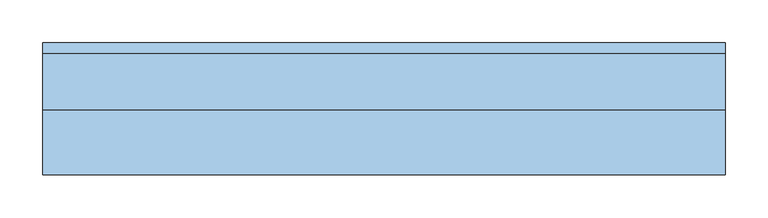
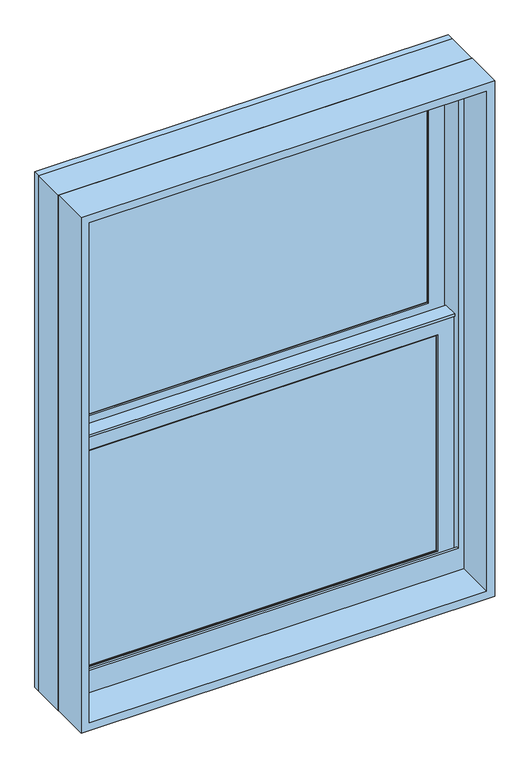
"""IFC4 building model written with IfcOpenShell, lengths in millimetres: window geometry, Window-Double_Hung-Marvin-Essential : ESDH2836."""

from ifc_helpers import new_model, si_unit, frame, origin, place, context, project, spatial, polyline, outline, extrude, faceted_brep, source, transform, mapped, element, save


def window_51e557a5(model_context):
    return source(origin(), model_context, "Body", "SolidModel", [
        extrude(outline(polyline([(123.825, 20.6375), (123.825, 15.875), (104.775, 15.875), (104.775, 20.6375), (123.825, 20.6375)])), frame((0.0, 0.0, 1441.45), z_axis=(0.0, 0.0, 1.0), x_axis=(1.0, 0.0, 0.0)), (0.0, 0.0, 1.0), 450.85),
        extrude(outline(polyline([(-104.775, 20.6375), (-104.775, 15.875), (-123.825, 15.875), (-123.825, 20.6375), (-104.775, 20.6375)])), frame((0.0, 0.0, 1441.45), z_axis=(0.0, 0.0, 1.0), x_axis=(1.0, 0.0, 0.0)), (0.0, 0.0, 1.0), 450.85),
        extrude(outline(polyline([(342.9, 20.6375), (342.9, 15.875), (-342.9, 15.875), (-342.9, 20.6375), (342.9, 20.6375)])), frame((0.0, 0.0, 1657.35), z_axis=(0.0, 0.0, 1.0), x_axis=(1.0, 0.0, 0.0)), (0.0, 0.0, 1.0), 19.05),
        extrude(outline(polyline([(-123.825, 46.83125), (-123.825, 51.59375), (-104.775, 51.59375), (-104.775, 46.83125), (-123.825, 46.83125)])), frame((0.0, 0.0, 1930.4), z_axis=(0.0, 0.0, 1.0), x_axis=(1.0, 0.0, 0.0)), (0.0, 0.0, 1.0), 450.85),
        extrude(outline(polyline([(104.775, 46.83125), (104.775, 51.59375), (123.825, 51.59375), (123.825, 46.83125), (104.775, 46.83125)])), frame((0.0, 0.0, 1930.4), z_axis=(0.0, 0.0, 1.0), x_axis=(1.0, 0.0, 0.0)), (0.0, 0.0, 1.0), 450.85),
        extrude(outline(polyline([(-342.9, 46.83125), (-342.9, 51.59375), (342.9, 51.59375), (342.9, 46.83125), (-342.9, 46.83125)])), frame((0.0, 0.0, 2146.3), z_axis=(0.0, 0.0, 1.0), x_axis=(1.0, 0.0, 0.0)), (0.0, 0.0, 1.0), 19.05),
        extrude(outline(polyline([(123.825, 20.6375), (104.775, 20.6375), (104.775, 25.4), (123.825, 25.4), (123.825, 20.6375)])), frame((0.0, 0.0, 1441.45), z_axis=(0.0, 0.0, 1.0), x_axis=(1.0, 0.0, 0.0)), (0.0, 0.0, 1.0), 450.85),
        extrude(outline(polyline([(-104.775, 20.6375), (-123.825, 20.6375), (-123.825, 25.4), (-104.775, 25.4), (-104.775, 20.6375)])), frame((0.0, 0.0, 1441.45), z_axis=(0.0, 0.0, 1.0), x_axis=(1.0, 0.0, 0.0)), (0.0, 0.0, 1.0), 450.85),
        extrude(outline(polyline([(342.9, 20.6375), (-342.9, 20.6375), (-342.9, 25.4), (342.9, 25.4), (342.9, 20.6375)])), frame((0.0, 0.0, 1657.35), z_axis=(0.0, 0.0, 1.0), x_axis=(1.0, 0.0, 0.0)), (0.0, 0.0, 1.0), 19.05),
        extrude(outline(polyline([(-123.825, 56.35625), (-104.775, 56.35625), (-104.775, 51.59375), (-123.825, 51.59375), (-123.825, 56.35625)])), frame((0.0, 0.0, 1930.4), z_axis=(0.0, 0.0, 1.0), x_axis=(1.0, 0.0, 0.0)), (0.0, 0.0, 1.0), 450.85),
        extrude(outline(polyline([(104.775, 56.35625), (123.825, 56.35625), (123.825, 51.59375), (104.775, 51.59375), (104.775, 56.35625)])), frame((0.0, 0.0, 1930.4), z_axis=(0.0, 0.0, 1.0), x_axis=(1.0, 0.0, 0.0)), (0.0, 0.0, 1.0), 450.85),
        extrude(outline(polyline([(-342.9, 56.35625), (342.9, 56.35625), (342.9, 51.59375), (-342.9, 51.59375), (-342.9, 56.35625)])), frame((0.0, 0.0, 2146.3), z_axis=(0.0, 0.0, 1.0), x_axis=(1.0, 0.0, 0.0)), (0.0, 0.0, 1.0), 19.05),
        faceted_brep([(-369.8875, 5.6780605, 1922.3351748), (-369.8875, 5.6780605, 1917.7), (369.8875, 5.6780605, 1917.7), (369.8875, 5.6780605, 1922.3351748), (-369.8875, 34.8118605, 1922.3351748), (369.8875, 34.8118605, 1922.3351748), (369.8875, 34.8118605, 1917.7), (-369.8875, 34.8118605, 1917.7), (-369.8875, 30.1625, 1917.7), (-369.8875, 30.1625, 1414.4625), (-369.8875, 8.9241104, 1414.4625), (-369.8875, 8.9241104, 1917.7), (369.8875, 8.9241104, 1917.7), (369.8875, 30.1625, 1917.7), (369.8875, 8.9241104, 1414.4625), (369.8875, 30.1625, 1414.4625), (-354.0034752, 11.90625, 1903.4034752), (-354.0034752, 30.1625, 1903.4034752), (354.0034752, 30.1625, 1903.4034752), (354.0034752, 11.90625, 1903.4034752), (-337.34375, 10.4662439, 1886.74375), (-337.34375, 11.90625, 1886.74375), (337.34375, 11.90625, 1886.74375), (337.34375, 10.4662439, 1886.74375), (338.8858834, 8.9241104, 1888.2858834), (-338.8858834, 8.9241104, 1888.2858834), (354.0034752, 30.1625, 1430.3465248), (354.0034752, 11.90625, 1430.3465248), (337.34375, 11.90625, 1447.00625), (337.34375, 10.4662439, 1447.00625), (338.8858834, 8.9241104, 1445.4641166), (-354.0034752, 30.1625, 1430.3465248), (-354.0034752, 11.90625, 1430.3465248), (-337.34375, 11.90625, 1447.00625), (-337.34375, 10.4662439, 1447.00625), (-338.8858834, 8.9241104, 1445.4641166)], [[[0, 1, 2, 3]], [[4, 5, 6, 7]], [[1, 0, 4, 7, 8, 9, 10, 11]], [[2, 1, 11, 12]], [[7, 6, 13, 8]], [[3, 2, 12, 14, 15, 13, 6, 5]], [[0, 3, 5, 4]], [[16, 17, 18, 19]], [[20, 21, 22, 23]], [[20, 23, 24, 25]], [[19, 18, 26, 27]], [[23, 22, 28, 29]], [[24, 23, 29, 30]], [[27, 26, 31, 32]], [[29, 28, 33, 34]], [[30, 29, 34, 35]], [[15, 14, 10, 9]], [[15, 9, 8, 13], [18, 17, 31, 26]], [[17, 16, 32, 31]], [[16, 19, 27, 32], [22, 21, 33, 28]], [[21, 20, 34, 33]], [[20, 25, 35, 34]], [[10, 14, 12, 11], [25, 24, 30, 35]]]),
        extrude(outline(polyline([(38.5955581, 1903.4125), (33.5778968, 1903.4125), (33.5778968, 1905.0), (39.9405976, 1905.0), (39.9405976, 1903.4125), (61.515625, 1903.4125), (47.6307501, 1900.0975159), (38.5955581, 1900.0975159), (38.5955581, 1903.4125)])), frame((-369.8875, 0.0, 0.0), z_axis=(1.0, 0.0, 0.0), x_axis=(0.0, 1.0, 0.0)), (0.0, 0.0, 1.0), 739.775),
        faceted_brep([(400.05, 0.0, 1384.3), (400.05, 0.0, 2438.4), (-400.05, 0.0, 2438.4), (-400.05, 0.0, 1384.3), (373.85625, 0.0, 1445.41875), (-373.85625, 0.0, 1445.41875), (-373.85625, 0.0, 2412.20625), (373.85625, 0.0, 2412.20625), (373.85625, 3.96875, 1384.3), (-373.85625, 3.96875, 1384.3), (-373.85625, 3.96875, 1445.41875), (373.85625, 3.96875, 1445.41875), (-400.05, 65.6828125, 1384.3), (-373.85625, 65.6828125, 1384.3), (373.85625, 65.6828125, 1384.3), (400.05, 65.6828125, 1384.3), (-400.05, 65.6828125, 2438.4), (400.05, 65.6828125, 2438.4), (373.85625, 65.6828125, 2412.20625), (-373.85625, 65.6828125, 2412.20625)], [[[0, 1, 2, 3], [4, 5, 6, 7]], [[8, 9, 10, 11]], [[5, 4, 11, 10]], [[0, 3, 12, 13, 9, 8, 14, 15]], [[13, 12, 16, 17, 15, 14, 18, 19]], [[13, 19, 6, 5, 10, 9]], [[7, 6, 19, 18]], [[18, 14, 8, 11, 4, 7]], [[1, 0, 15, 17]], [[2, 1, 17, 16]], [[3, 2, 16, 12]]]),
        faceted_brep([(373.85625, 30.1625, 1911.35), (372.26875, 30.1625, 1911.35), (372.26875, 30.1625, 1408.6544613), (373.85625, 30.1625, 1408.6544613), (-372.26875, 30.1625, 1911.35), (-373.85625, 30.1625, 1911.35), (-373.85625, 30.1625, 1408.6544613), (-372.26875, 30.1625, 1408.6544613), (372.26875, 63.5, 1911.35), (373.85625, 63.5, 1911.35), (373.85625, 63.5, 1402.1743077), (372.26875, 63.5, 1402.1743077), (-373.85625, 63.5, 1911.35), (-372.26875, 63.5, 1911.35), (-372.26875, 63.5, 1402.1743077), (-373.85625, 63.5, 1402.1743077), (385.1108932, 3.96875, 1413.7460105), (385.1108932, 3.96875, 1384.3), (385.1108932, 65.6828125, 1384.3), (385.1108932, 65.6828125, 1401.750012), (-385.1108932, 3.96875, 1384.3), (-385.1108932, 3.96875, 1413.7460105), (-385.1108932, 65.6828125, 1401.750012), (-385.1108932, 65.6828125, 1384.3), (385.1108932, 78.58125, 1399.2428097), (-385.1108932, 78.58125, 1399.2428097), (-383.0971252, 68.2348864, 1401.2539391), (-365.13135, 68.2348864, 1401.2539391), (-365.13135, 65.6828125, 1401.750012), (365.13135, 65.6828125, 1401.750012), (365.13135, 68.2348864, 1401.2539391), (383.0971252, 68.2348864, 1401.2539391), (-400.05, 65.6828125, 1384.3), (-400.05, 78.5948249, 1384.3), (400.05, 78.5948249, 1384.3), (400.05, 65.6828125, 1384.3), (-400.05, 78.58125, 2438.4), (400.05, 78.58125, 2438.4), (385.1108932, 78.58125, 2423.4608932), (-385.1108932, 78.58125, 2423.4608932), (-400.05, 65.6828125, 2438.4), (-383.0971252, 68.2348864, 2421.4471252), (383.0971252, 68.2348864, 2421.4471252), (365.13135, 68.2348864, 2403.48135), (-365.13135, 68.2348864, 2403.48135), (-365.13135, 65.6828125, 2403.48135), (365.13135, 65.6828125, 2403.48135), (400.05, 65.6828125, 2438.4)], [[[0, 1, 2, 3]], [[4, 5, 6, 7]], [[8, 9, 10, 11]], [[12, 13, 14, 15]], [[1, 8, 11, 2]], [[9, 0, 3, 10]], [[1, 0, 9, 8]], [[5, 4, 13, 12]], [[5, 12, 15, 6]], [[13, 4, 7, 14]], [[16, 17, 18, 19]], [[20, 21, 22, 23]], [[24, 25, 26, 27, 28, 22, 21, 16, 19, 29, 30, 31], [3, 2, 11, 10], [7, 6, 15, 14]], [[17, 16, 21, 20]], [[17, 20, 23, 32, 33, 34, 35, 18]], [[34, 33, 36, 37], [25, 24, 38, 39]], [[33, 32, 40, 36]], [[39, 41, 26, 25]], [[41, 42, 31, 30, 43, 44, 27, 26]], [[44, 45, 28, 27]], [[40, 32, 23, 22, 28, 45, 46, 29, 19, 18, 35, 47]], [[36, 40, 47, 37]], [[39, 38, 42, 41]], [[44, 43, 46, 45]], [[34, 37, 47, 35]], [[42, 38, 24, 31]], [[46, 43, 30, 29]]]),
        extrude(outline(polyline([(350.04375, 11.90625), (-350.04375, 11.90625), (-350.04375, 15.08125), (350.04375, 15.08125), (350.04375, 11.90625)])), frame((0.0, 0.0, 1434.30625), z_axis=(0.0, 0.0, 1.0), x_axis=(1.0, 0.0, 0.0)), (0.0, 0.0, 1.0), 465.1375),
        extrude(outline(polyline([(350.04375, 42.8625), (-350.04375, 42.8625), (-350.04375, 46.0375), (350.04375, 46.0375), (350.04375, 42.8625)])), frame((0.0, 0.0, 1923.25625), z_axis=(0.0, 0.0, 1.0), x_axis=(1.0, 0.0, 0.0)), (0.0, 0.0, 1.0), 465.1375),
        faceted_brep([(-337.34375, 31.194477, 1886.74375), (-338.8858834, 32.7366104, 1888.2858834), (338.8858834, 32.7366104, 1888.2858834), (337.34375, 31.194477, 1886.74375), (-337.34375, 30.1625, 1886.74375), (337.34375, 30.1625, 1886.74375), (-369.8875, 32.7366104, 1919.2875), (-369.8875, 30.1625, 1919.2875), (369.8875, 30.1625, 1919.2875), (369.8875, 32.7366104, 1919.2875), (338.8858834, 32.7366104, 1445.4641166), (337.34375, 31.194477, 1447.00625), (337.34375, 30.1625, 1447.00625), (369.8875, 30.1625, 1414.4625), (369.8875, 32.7366104, 1414.4625), (-338.8858834, 32.7366104, 1445.4641166), (-337.34375, 31.194477, 1447.00625), (-337.34375, 30.1625, 1447.00625), (-369.8875, 30.1625, 1414.4625), (-369.8875, 32.7366104, 1414.4625)], [[[0, 1, 2, 3]], [[4, 0, 3, 5]], [[6, 7, 8, 9]], [[3, 2, 10, 11]], [[5, 3, 11, 12]], [[9, 8, 13, 14]], [[11, 10, 15, 16]], [[12, 11, 16, 17]], [[14, 13, 18, 19]], [[9, 14, 19, 6], [1, 15, 10, 2]], [[16, 15, 1, 0]], [[17, 16, 0, 4]], [[7, 18, 13, 8], [5, 12, 17, 4]], [[19, 18, 7, 6]]]),
        faceted_brep([(-354.0034752, 42.8625, 2392.3534752), (-354.0034752, 61.11875, 2392.3534752), (354.0034752, 61.11875, 2392.3534752), (354.0034752, 42.8625, 2392.3534752), (-337.34375, 41.4224939, 2375.69375), (-337.34375, 42.8625, 2375.69375), (337.34375, 42.8625, 2375.69375), (337.34375, 41.4224939, 2375.69375), (-338.8858834, 39.8803604, 2377.2358834), (338.8858834, 39.8803604, 2377.2358834), (-369.8875, 61.11875, 2408.2375), (-369.8875, 39.8803604, 2408.2375), (369.8875, 39.8803604, 2408.2375), (369.8875, 61.11875, 2408.2375), (354.0034752, 61.11875, 1919.2965248), (354.0034752, 42.8625, 1919.2965248), (337.34375, 42.8625, 1935.95625), (337.34375, 41.4224939, 1935.95625), (338.8858834, 39.8803604, 1934.4141166), (369.8875, 39.8803604, 1903.4125), (369.8875, 61.11875, 1903.4125), (-354.0034752, 61.11875, 1919.2965248), (-354.0034752, 42.8625, 1919.2965248), (-337.34375, 42.8625, 1935.95625), (-337.34375, 41.4224939, 1935.95625), (-338.8858834, 39.8803604, 1934.4141166), (-369.8875, 39.8803604, 1903.4125), (-369.8875, 61.11875, 1903.4125)], [[[0, 1, 2, 3]], [[4, 5, 6, 7]], [[8, 4, 7, 9]], [[10, 11, 12, 13]], [[3, 2, 14, 15]], [[7, 6, 16, 17]], [[9, 7, 17, 18]], [[13, 12, 19, 20]], [[15, 14, 21, 22]], [[17, 16, 23, 24]], [[18, 17, 24, 25]], [[20, 19, 26, 27]], [[13, 20, 27, 10], [1, 21, 14, 2]], [[22, 21, 1, 0]], [[3, 15, 22, 0], [5, 23, 16, 6]], [[24, 23, 5, 4]], [[25, 24, 4, 8]], [[11, 26, 19, 12], [9, 18, 25, 8]], [[27, 26, 11, 10]]]),
        faceted_brep([(-369.8875, 61.11875, 1903.4125), (-369.8875, 63.6928604, 1903.4125), (369.8875, 63.6928604, 1903.4125), (369.8875, 61.11875, 1903.4125), (-337.34375, 62.150727, 1935.95625), (-337.34375, 61.11875, 1935.95625), (337.34375, 61.11875, 1935.95625), (337.34375, 62.150727, 1935.95625), (-338.8858834, 63.6928604, 1934.4141166), (338.8858834, 63.6928604, 1934.4141166), (369.8875, 63.6928604, 2408.2375), (369.8875, 61.11875, 2408.2375), (337.34375, 61.11875, 2375.69375), (337.34375, 62.150727, 2375.69375), (338.8858834, 63.6928604, 2377.2358834), (-369.8875, 63.6928604, 2408.2375), (-369.8875, 61.11875, 2408.2375), (-337.34375, 61.11875, 2375.69375), (-337.34375, 62.150727, 2375.69375), (-338.8858834, 63.6928604, 2377.2358834)], [[[0, 1, 2, 3]], [[4, 5, 6, 7]], [[8, 4, 7, 9]], [[3, 2, 10, 11]], [[7, 6, 12, 13]], [[9, 7, 13, 14]], [[11, 10, 15, 16]], [[13, 12, 17, 18]], [[14, 13, 18, 19]], [[16, 15, 1, 0]], [[3, 11, 16, 0], [5, 17, 12, 6]], [[18, 17, 5, 4]], [[19, 18, 4, 8]], [[1, 15, 10, 2], [9, 14, 19, 8]]]),
        extrude(outline(polyline([(350.04375, 26.19375), (-350.04375, 26.19375), (-350.04375, 30.1625), (350.04375, 30.1625), (350.04375, 26.19375)])), frame((0.0, 0.0, 1434.30625), z_axis=(0.0, 0.0, 1.0), x_axis=(1.0, 0.0, 0.0)), (0.0, 0.0, 1.0), 465.1375),
        extrude(outline(polyline([(350.04375, 57.15), (-350.04375, 57.15), (-350.04375, 61.11875), (350.04375, 61.11875), (350.04375, 57.15)])), frame((0.0, 0.0, 1923.25625), z_axis=(0.0, 0.0, 1.0), x_axis=(1.0, 0.0, 0.0)), (0.0, 0.0, 1.0), 465.1375),
        extrude(outline(polyline([(2438.4, 400.05), (2438.4, -400.05), (1384.3, -400.05), (1384.3, 400.05), (2438.4, 400.05)]), holes=[polyline([(2422.525, 384.175), (1400.175, 384.175), (1400.175, -384.175), (2422.525, -384.175), (2422.525, 384.175)])]), frame((0.0, -76.2, 0.0), z_axis=(0.0, 1.0, 0.0), x_axis=(0.0, 0.0, 1.0)), (0.0, 0.0, 1.0), 75.40625),
    ])


if __name__ == "__main__":
    model = new_model("IFC4")
    model_context = context("Model", 3, world=origin())
    ifc_project = project(units=[si_unit("LENGTHUNIT", "METRE", prefix="MILLI")], contexts=[model_context])
    site = spatial("IfcSite", under=ifc_project)
    building = spatial("IfcBuilding", under=site)
    placement = place(None, origin())
    window_shape = window_51e557a5(model_context)
    element("IfcWindow", 1, ObjectType="Window-Double_Hung-Marvin-Essential : ESDH2836", at=placement, inside=building, context=model_context, shape_type="MappedRepresentation", body=[
        mapped(window_shape, transform((0.0, 0.0, 0.0), x_axis=(1.0, 0.0, 0.0), y_axis=(0.0, 1.0, 0.0), z_axis=(0.0, 0.0, 1.0))),
    ])
    save(model, "model.ifc")

# Revit data of these elements
# Type "Window-Double_Hung-Marvin-Essential : ESDH2836"
#   Type Mark = "43"
#   Window Type = "Essential Double Hung"
#   Product data url = "https://bimobject.com/marvin-windows-and-doors/product/marvin-dhwau"
#   Product Guid = "c4a96547-874c-4385-91dc-a058adc19d98"
#   Frame = "All Ultrex"
#   Egress Window = "No"
#   URL = "www.marvin.com"
#   Model = "ESDH2836"
#   Manufacturer = "Marvin Windows and Doors"
#   Label Egress = ""
#   Glass Type = "IG Low E II with Argon"
#   Design Pressure = "DP50"
#   Description = "3242 DBHG"
#   Analytic Construction = "<None>"
#   Prairie Corner Width = 0' - 4"
#   Prairie Corner Height = 0' - 4"
#   Egress Width = 2' - 4 9/16"
#   Egress Height = 1' - 4 27/128"
#   Rough Width = 2' - 8"
#   Rough Height = 3' - 6"
#   Nominal Width = 2' - 8"
#   Nominal Height = 3' - 6"
#   Inset to Installation Flange [instance default] = 0' - 1"
#   Height = 3' - 5 1/2"
#   Egress Area = 3.21545 SF
#   Default Head Height = 8' - 0"
#   Width = 2' - 7 1/2"
#   Daylight Area = 6.38699 SF
#   DLO Width = 2' - 2 9/16"
#   DLO Height = 1' - 5 5/16"
#   Muntins Top Sash = yes
#   Lites Wide Top Sash = 3
#   Lites Wide Bottom Sash = 3
#   Lites High Top Sash = 2
#   Lites High Bottom Sash = 2
#   Lite Cut Prairie 9 = no
#   Lite Cut HV Grid = yes
#   Muntins Bottom Sash = yes
#   Label Visibility = no
#   Jamb Extension Visibility = yes
#   Edition number = 1
#   Interior Material = Ultrex-Marvin-Stonewhite
#   Glazing Material = Glass-Marvin-IG Low E II with Argon
#   Cladding Material = Ultrex-Marvin-Pebblegray
#   Wall Closure = (empty or 0)
#   Assembly Code = ""
# Element 1 (IfcWindow, "Window-Double_Hung-Marvin-Essential : ESDH2836")
#   Materials on its faces: "Ultrex-Marvin-Pebblegray", "Ultrex-Marvin-Stonewhite", "Glass-Marvin-IG Low E II with Argon"
# Materials
#   "Ultrex-Marvin-Stonewhite": class "Paint", colour RGB 250 251 245, transparency 0
#   "Glass-Marvin-IG Low E II with Argon": class "Glass", colour RGB 0 128 192, transparency 0.85
#   "Ultrex-Marvin-Pebblegray": class "Paint", colour RGB 189 185 173, transparency 0
